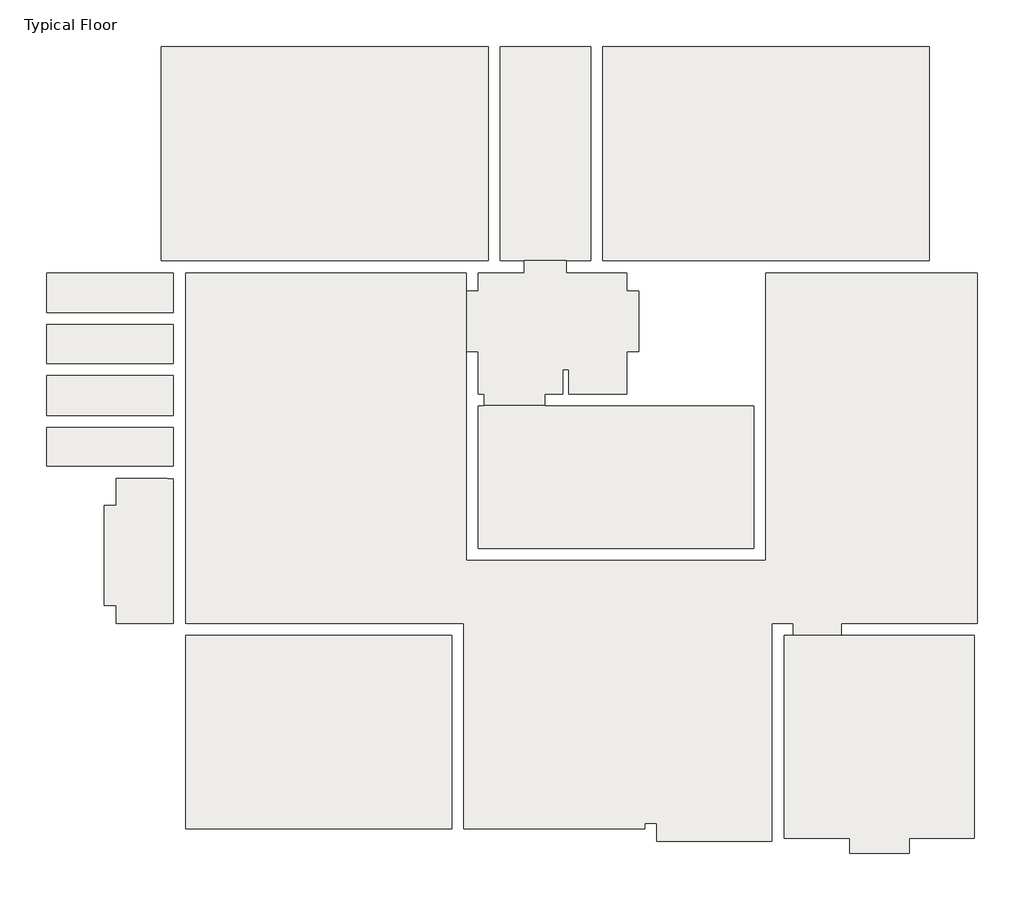
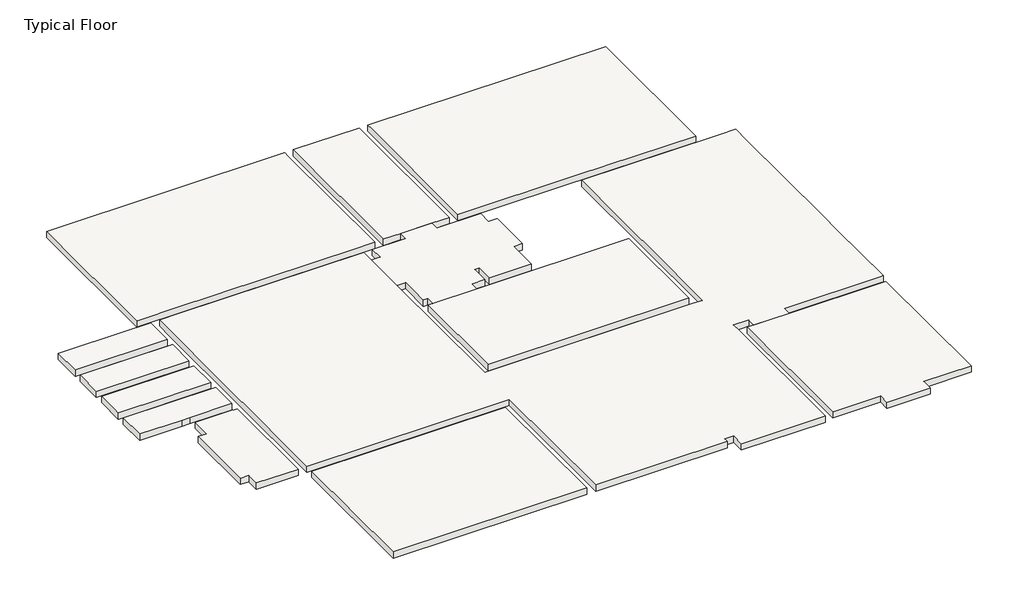
# One storey: 13 slabs.
"""IFC4 building model written with IfcOpenShell, lengths in millimetres."""

from ifc_helpers import new_model, si_unit, frame, origin, place, context, project, spatial, polyline, outline, extrude, faceted_brep, element, save

model = new_model("IFC4")

# Units and contexts
model_context = context("Model", 3, world=origin())
ifc_project = project(units=[si_unit("LENGTHUNIT", "METRE", prefix="MILLI")], contexts=[model_context])

# Site, building, storey
site = spatial("IfcSite", under=ifc_project)
building = spatial("IfcBuilding", under=site)
storey = spatial("IfcBuildingStorey", under=building, Name="Typical Floor", Elevation=3000.0)

# Slabs
placement = place(None, origin())
element("IfcSlab", 1, ObjectType="15", at=placement, inside=storey, context=model_context, shape_type="Brep", body=[
    faceted_brep([(623.0052446, -1951.586272, 2850.0), (623.0052446, 1403.8860569, 2850.0), (773.8332228, 1403.8860569, 2850.0), (1572.9542214, 1403.8860569, 2850.0), (3773.240421, 1403.8860569, 2850.0), (3773.240421, -1951.586272, 2850.0), (2697.5461186, -1951.586272, 2850.0), (2697.5461186, -2201.586272, 2850.0), (1713.8332228, -2201.586272, 2850.0), (1713.8332228, -1951.586272, 2850.0), (623.0052446, 1403.8860569, 3000.0), (623.0052446, -1951.586272, 3000.0), (1713.8332228, -1951.586272, 3000.0), (1713.8332228, -2201.586272, 3000.0), (2697.5461186, -2201.586272, 3000.0), (2697.5461186, -1951.586272, 3000.0), (3773.240421, -1951.586272, 3000.0), (3773.240421, 1403.8860569, 3000.0), (1572.9542214, 1403.8860569, 3000.0), (773.8332228, 1403.8860569, 3000.0)], [[[0, 1, 2, 3, 4, 5, 6, 7, 8, 9]], [[10, 11, 12, 13, 14, 15, 16, 17, 18, 19]], [[1, 0, 11, 10]], [[4, 3, 2, 1, 10, 19, 18, 17]], [[5, 4, 17, 16]], [[0, 9, 12, 11]], [[6, 5, 16, 15]], [[7, 6, 15, 14]], [[8, 7, 14, 13]], [[9, 8, 13, 12]]]),
])
element("IfcSlab", 2, ObjectType="15", at=placement, inside=storey, context=model_context, shape_type="SweptSolid", body=[
    extrude(outline(polyline([(-4877.1268931, 1403.8855607), (-4877.1268931, -1797.4530794), (-9277.1472957, -1797.4530794), (-9277.1472957, 1403.8855607), (-4877.1268931, 1403.8855607)])), frame((0.0, 0.0, 2850.0), z_axis=(0.0, 0.0, 1.0), x_axis=(1.0, 0.0, 0.0)), (0.0, 0.0, 1.0), 150.0),
])
element("IfcSlab", 3, ObjectType="15", at=placement, inside=storey, context=model_context, shape_type="SweptSolid", body=[
    extrude(outline(polyline([(123.9972875, 2842.5882386), (-4436.0027125, 2842.5882386), (-4436.0027125, 5202.5780208), (-4335.7799232, 5202.5780208), (-4335.7799232, 5207.5780373), (-3335.5551136, 5207.5780373), (-3335.5551136, 5202.5780373), (123.9972875, 5202.5780373), (123.9972875, 2842.5882386)])), frame((0.0, 0.0, 2850.0), z_axis=(0.0, 0.0, 1.0), x_axis=(1.0, 0.0, 0.0)), (0.0, 0.0, 1.0), 150.0),
])
element("IfcSlab", 4, ObjectType="15", at=placement, inside=storey, context=model_context, shape_type="Brep", body=[
    faceted_brep([(-11576.8844551, 4205.5532536, 2850.0), (-11576.8844551, 4845.5532536, 2850.0), (-9476.8844551, 4845.5532536, 2850.0), (-9476.8844551, 4297.7532903, 2850.0), (-9476.8844551, 4205.5532536, 2850.0), (-10423.025528, 4205.5532536, 2850.0), (-10423.025528, 4208.1905626, 2850.0), (-10623.025528, 4208.1905626, 2850.0), (-10623.025528, 4205.5532536, 2850.0), (-11576.8844551, 4845.5532536, 3000.0), (-11576.8844551, 4205.5532536, 3000.0), (-10623.025528, 4205.5532536, 3000.0), (-10623.025528, 4208.1905626, 3000.0), (-10423.025528, 4208.1905626, 3000.0), (-10423.025528, 4205.5532536, 3000.0), (-9476.8844551, 4205.5532536, 3000.0), (-9476.8844551, 4297.7532903, 3000.0), (-9476.8844551, 4845.5532536, 3000.0)], [[[0, 1, 2, 3, 4, 5, 6, 7, 8]], [[9, 10, 11, 12, 13, 14, 15, 16, 17]], [[15, 4, 3, 2, 17, 16]], [[4, 15, 14, 5]], [[10, 0, 8, 11]], [[1, 0, 10, 9]], [[2, 1, 9, 17]], [[13, 6, 5, 14]], [[7, 12, 11, 8]], [[12, 7, 6, 13]]]),
])
element("IfcSlab", 5, ObjectType="15", at=placement, inside=storey, context=model_context, shape_type="SweptSolid", body=[
    extrude(outline(polyline([(-9476.8844551, 5705.5532536), (-9476.8844551, 5045.5532536), (-11576.8844551, 5045.5532536), (-11576.8844551, 5705.5532536), (-9476.8844551, 5705.5532536)])), frame((0.0, 0.0, 2850.0), z_axis=(0.0, 0.0, 1.0), x_axis=(1.0, 0.0, 0.0)), (0.0, 0.0, 1.0), 150.0),
])
element("IfcSlab", 6, ObjectType="15", at=placement, inside=storey, context=model_context, shape_type="SweptSolid", body=[
    extrude(outline(polyline([(-9476.8844551, 6545.5532536), (-9476.8844551, 5905.5532536), (-11576.8844551, 5905.5532536), (-11576.8844551, 6545.5532536), (-9476.8844551, 6545.5532536)])), frame((0.0, 0.0, 2850.0), z_axis=(0.0, 0.0, 1.0), x_axis=(1.0, 0.0, 0.0)), (0.0, 0.0, 1.0), 150.0),
])
element("IfcSlab", 7, ObjectType="15", at=placement, inside=storey, context=model_context, shape_type="Brep", body=[
    faceted_brep([(-9476.8844551, 7405.5532536, 2850.0), (-9476.8844551, 6745.5532536, 2850.0), (-11576.8844551, 6745.5532536, 2850.0), (-11576.8844551, 7405.5532536, 2850.0), (-9476.8844551, 7405.5532536, 3000.0), (-9682.6961091, 7405.5532536, 3000.0), (-9932.6961091, 7405.5532536, 3000.0), (-11576.8844551, 7405.5532536, 3000.0), (-11576.8844551, 6745.5532536, 3000.0), (-9476.8844551, 6745.5532536, 3000.0), (-9476.8844551, 7005.5532536, 3000.0)], [[[0, 1, 2, 3]], [[4, 5, 6, 7, 8, 9, 10]], [[1, 0, 4, 10, 9]], [[2, 1, 9, 8]], [[3, 2, 8, 7]], [[0, 3, 7, 6, 5, 4]]]),
])
element("IfcSlab", 8, ObjectType="15", at=placement, inside=storey, context=model_context, shape_type="Brep", body=[
    faceted_brep([(3026.9297982, 11151.9234339, 2850.0), (3026.9297982, 7605.5532536, 2850.0), (-2375.600893, 7605.5532536, 2850.0), (-2375.600893, 11151.9234339, 2850.0), (3026.9297982, 11151.9234339, 3000.0), (-2375.600893, 11151.9234339, 3000.0), (-2375.600893, 11003.3317688, 3000.0), (-2375.600893, 7605.5532536, 3000.0), (323.9972875, 7605.5532536, 3000.0), (3026.9297982, 7605.5532536, 3000.0), (3026.9297982, 11001.5732233, 3000.0)], [[[0, 1, 2, 3]], [[4, 5, 6, 7, 8, 9, 10]], [[1, 0, 4, 10, 9]], [[2, 1, 9, 8, 7]], [[3, 2, 7, 6, 5]], [[0, 3, 5, 4]]]),
])
element("IfcSlab", 9, ObjectType="15", at=placement, inside=storey, context=model_context, shape_type="Brep", body=[
    faceted_brep([(-2575.600893, 11151.9234339, 2850.0), (-2575.600893, 7605.5532536, 2850.0), (-2975.6858924, 7605.5532536, 2850.0), (-3676.9016865, 7605.5532536, 2850.0), (-4072.3731245, 7605.5532536, 2850.0), (-4072.3731245, 11151.9234339, 2850.0), (-2575.600893, 11151.9234339, 3000.0), (-4072.3731245, 11151.9234339, 3000.0), (-4072.3731245, 11003.3317688, 3000.0), (-4072.3731245, 7605.5532536, 3000.0), (-3676.9016865, 7605.5532536, 3000.0), (-2975.6858924, 7605.5532536, 3000.0), (-2575.600893, 7605.5532536, 3000.0), (-2575.600893, 11003.3317688, 3000.0)], [[[0, 1, 2, 3, 4, 5]], [[6, 7, 8, 9, 10, 11, 12, 13]], [[1, 0, 6, 13, 12]], [[4, 3, 2, 1, 12, 11, 10, 9]], [[5, 4, 9, 8, 7]], [[0, 5, 7, 6]]]),
])
element("IfcSlab", 10, ObjectType="15", at=placement, inside=storey, context=model_context, shape_type="Brep", body=[
    faceted_brep([(-4272.3731245, 11151.9234339, 2850.0), (-4272.3731245, 7605.5532536, 2850.0), (-9682.6961091, 7605.5532536, 2850.0), (-9682.6961091, 11151.9234339, 2850.0), (-4272.3731245, 11151.9234339, 3000.0), (-9682.6961091, 11151.9234339, 3000.0), (-9682.6961091, 11001.5732233, 3000.0), (-9682.6961091, 7605.5532536, 3000.0), (-9476.8844551, 7605.5532536, 3000.0), (-8876.8844551, 7605.5532536, 3000.0), (-4636.0027125, 7605.5532536, 3000.0), (-4436.0027125, 7605.5532536, 3000.0), (-4272.3731245, 7605.5532536, 3000.0), (-4272.3731245, 11003.3317688, 3000.0)], [[[0, 1, 2, 3]], [[4, 5, 6, 7, 8, 9, 10, 11, 12, 13]], [[1, 0, 4, 13, 12]], [[2, 1, 12, 11, 10, 9, 8, 7]], [[3, 2, 7, 6, 5]], [[0, 3, 5, 4]]]),
])
element("IfcSlab", 11, ObjectType="15", at=placement, inside=storey, context=model_context, shape_type="SweptSolid", body=[
    extrude(outline(polyline([(-2975.6858924, 7605.5532536), (-2975.6858924, 7405.5532536), (-1977.004444, 7405.5532536), (-1977.004444, 7102.4758421), (-1777.004444, 7102.4758421), (-1777.004444, 6104.8971794), (-1977.004444, 6104.8971794), (-1977.004444, 5402.5780373), (-2935.9943496, 5402.5780373), (-2935.9943496, 5803.2422484), (-3035.9943496, 5803.2422484), (-3035.9943496, 5402.5780373), (-3335.5551136, 5402.5780373), (-3335.5551136, 5207.5780373), (-4335.7799232, 5207.5780373), (-4335.7799232, 5402.5780208), (-4436.0027125, 5402.5780208), (-4436.0027125, 6102.5882386), (-4636.0027125, 6102.5882386), (-4636.0027125, 7102.4759909), (-4436.0027125, 7102.4759909), (-4436.0027125, 7405.5532536), (-3676.9016865, 7405.5532536), (-3676.9016865, 7605.5532536), (-2975.6858924, 7605.5532536)])), frame((0.0, 0.0, 2850.0), z_axis=(0.0, 0.0, 1.0), x_axis=(1.0, 0.0, 0.0)), (0.0, 0.0, 1.0), 150.0),
])
element("IfcSlab", 12, ObjectType="15", at=placement, inside=storey, context=model_context, shape_type="Brep", body=[
    faceted_brep([(323.9972875, 2642.5882386, 2850.0), (323.9972875, 7405.5532536, 2850.0), (3423.240421, 7405.5532536, 2850.0), (3823.240421, 7405.5532536, 2850.0), (3823.240421, 7005.5532536, 2850.0), (3823.240421, 1603.8858088, 2850.0), (3773.240421, 1603.8858088, 2850.0), (1572.9542214, 1603.8858088, 2850.0), (1572.9542214, 1403.8858088, 2850.0), (773.8332228, 1403.8858088, 2850.0), (773.8332228, 1603.8860569, 2850.0), (423.0052446, 1603.8860569, 2850.0), (423.0052446, 1403.8860569, 2850.0), (423.0052446, -2001.586272, 2850.0), (-1481.0647566, -2001.586272, 2850.0), (-1481.0647566, -1701.586272, 2850.0), (-1681.0647566, -1701.586272, 2850.0), (-1681.0647566, -1797.4530794, 2850.0), (-4677.1268931, -1797.4530794, 2850.0), (-4677.1268931, 1603.8855607, 2850.0), (-4877.1268931, 1603.8855607, 2850.0), (-9276.8844551, 1603.8855607, 2850.0), (-9276.8844551, 7005.5532536, 2850.0), (-9276.8844551, 7405.5532536, 2850.0), (-8876.8844551, 7405.5532536, 2850.0), (-4636.0027125, 7405.5532536, 2850.0), (-4636.0027125, 7102.4759909, 2850.0), (-4636.0027125, 6102.5882386, 2850.0), (-4636.0027125, 2842.5882386, 2850.0), (-4636.0027125, 2642.5882386, 2850.0), (123.9972875, 2642.5882386, 2850.0), (323.9972875, 7405.5532536, 3000.0), (323.9972875, 2642.5882386, 3000.0), (123.9972875, 2642.5882386, 3000.0), (-4636.0027125, 2642.5882386, 3000.0), (-4636.0027125, 2842.5882386, 3000.0), (-4636.0027125, 6102.5882386, 3000.0), (-4636.0027125, 7102.4759909, 3000.0), (-4636.0027125, 7405.5532536, 3000.0), (-8876.8844551, 7405.5532536, 3000.0), (-9276.8844551, 7405.5532536, 3000.0), (-9276.8844551, 7005.5532536, 3000.0), (-9276.8844551, 4297.7532903, 3000.0), (-9276.8844551, 3997.7532903, 3000.0), (-9276.8844551, 1603.8855607, 3000.0), (-4877.1268931, 1603.8855607, 3000.0), (-4677.1268931, 1603.8855607, 3000.0), (-4677.1268931, -1797.4530794, 3000.0), (-1681.0647566, -1797.4530794, 3000.0), (-1681.0647566, -1701.586272, 3000.0), (-1481.0647566, -1701.586272, 3000.0), (-1481.0647566, -2001.586272, 3000.0), (423.0052446, -2001.586272, 3000.0), (423.0052446, 1403.8860569, 3000.0), (423.0052446, 1603.8860569, 3000.0), (773.8332228, 1603.8860569, 3000.0), (773.8332228, 1403.8858088, 3000.0), (1572.9542214, 1403.8858088, 3000.0), (1572.9542214, 1603.8858088, 3000.0), (3773.240421, 1603.8858088, 3000.0), (3823.240421, 1603.8858088, 3000.0), (3823.240421, 3398.9311809, 3000.0), (3823.240421, 3998.9311809, 3000.0), (3823.240421, 7005.5532536, 3000.0), (3823.240421, 7405.5532536, 3000.0), (3423.240421, 7405.5532536, 3000.0)], [[[0, 1, 2, 3, 4, 5, 6, 7, 8, 9, 10, 11, 12, 13, 14, 15, 16, 17, 18, 19, 20, 21, 22, 23, 24, 25, 26, 27, 28, 29, 30]], [[31, 32, 33, 34, 35, 36, 37, 38, 39, 40, 41, 42, 43, 44, 45, 46, 47, 48, 49, 50, 51, 52, 53, 54, 55, 56, 57, 58, 59, 60, 61, 62, 63, 64, 65]], [[34, 29, 28, 27, 26, 25, 38, 37, 36, 35]], [[29, 34, 33, 32, 0, 30]], [[1, 0, 32, 31]], [[1, 31, 65, 64, 3, 2]], [[3, 64, 63, 62, 61, 60, 5, 4]], [[5, 60, 59, 58, 7, 6]], [[8, 7, 58, 57]], [[9, 8, 57, 56]], [[10, 9, 56, 55]], [[11, 10, 55, 54]], [[11, 54, 53, 52, 13, 12]], [[14, 13, 52, 51]], [[15, 14, 51, 50]], [[16, 15, 50, 49]], [[17, 16, 49, 48]], [[18, 17, 48, 47]], [[19, 18, 47, 46]], [[19, 46, 45, 44, 21, 20]], [[21, 44, 43, 42, 41, 40, 23, 22]], [[23, 40, 39, 38, 25, 24]]]),
])
element("IfcSlab", 13, ObjectType="15", at=placement, inside=storey, context=model_context, shape_type="Brep", body=[
    faceted_brep([(-9476.8844551, 1603.8855607, 2850.0), (-10423.025528, 1603.8855607, 2850.0), (-10423.025528, 1900.4395709, 2850.0), (-10623.025528, 1900.4395709, 2850.0), (-10623.025528, 3558.1905626, 2850.0), (-10423.025528, 3558.1905626, 2850.0), (-10423.025528, 4005.5532536, 2850.0), (-9576.8844551, 4005.5532536, 2850.0), (-9576.8844551, 3997.7532903, 2850.0), (-9476.8844551, 3997.7532903, 2850.0), (-10423.025528, 1603.8855607, 3000.0), (-9477.1472957, 1603.8855607, 3000.0), (-9476.8844551, 1603.8855607, 3000.0), (-9476.8844551, 3997.7532903, 3000.0), (-9576.8844551, 3997.7532903, 3000.0), (-9576.8844551, 4005.5532536, 3000.0), (-10423.025528, 4005.5532536, 3000.0), (-10423.025528, 3558.1905626, 3000.0), (-10623.025528, 3558.1905626, 3000.0), (-10623.025528, 1900.4395709, 3000.0), (-10423.025528, 1900.4395709, 3000.0)], [[[0, 1, 2, 3, 4, 5, 6, 7, 8, 9]], [[10, 11, 12, 13, 14, 15, 16, 17, 18, 19, 20]], [[12, 0, 9, 13]], [[1, 0, 12, 11, 10]], [[2, 1, 10, 20]], [[3, 2, 20, 19]], [[4, 3, 19, 18]], [[5, 4, 18, 17]], [[6, 5, 17, 16]], [[6, 16, 15, 7]], [[8, 14, 13, 9]], [[14, 8, 7, 15]]]),
])

save(model, "model.ifc")

# Revit data of these elements
# Type "15"
#   Function = 0
#   Layers, outside or top first: 15 cm "Concrete" (function 1)
# Element 1 (IfcSlab, "15")
#   Mark = "S1"
#   SOFiSTiK_AMG_Comments = ""
#   built-in parameter 1001955 = 3.14159 (stored number, unit not read)
#   Height Offset From Level = 0 cm
#   built-in parameter 1001954 = 1
#   SOFiSTiK_AMG_Scheduled = yes
#   SOFiSTiK_AMG_Adjusted = yes
#   Phase Created = New Construction
#   Materials on its faces: "Concrete"
# Element 2 (IfcSlab, "15")
#   Mark = "S2"
#   SOFiSTiK_AMG_Comments = ""
#   Height Offset From Level = 0 cm
#   built-in parameter 1001954 = 1
#   SOFiSTiK_AMG_Scheduled = yes
#   SOFiSTiK_AMG_Adjusted = yes
#   Phase Created = New Construction
#   Materials on its faces: "Concrete"
# Element 3 (IfcSlab, "15")
#   Mark = "S3"
#   SOFiSTiK_AMG_Comments = ""
#   Height Offset From Level = 0 cm
#   built-in parameter 1001954 = 1
#   SOFiSTiK_AMG_Scheduled = yes
#   SOFiSTiK_AMG_Adjusted = yes
#   Phase Created = New Construction
#   Materials on its faces: "Concrete"
# Element 4 (IfcSlab, "15")
#   Mark = "S4"
#   SOFiSTiK_AMG_Comments = ""
#   Height Offset From Level = 0 cm
#   built-in parameter 1001954 = 1
#   SOFiSTiK_AMG_Scheduled = yes
#   SOFiSTiK_AMG_Adjusted = yes
#   Phase Created = New Construction
#   Materials on its faces: "Concrete"
# Element 5 (IfcSlab, "15")
#   Mark = "S5"
#   SOFiSTiK_AMG_Comments = ""
#   Height Offset From Level = 0 cm
#   built-in parameter 1001954 = 1
#   SOFiSTiK_AMG_Scheduled = yes
#   SOFiSTiK_AMG_Adjusted = yes
#   Phase Created = New Construction
#   Materials on its faces: "Concrete"
# Element 6 (IfcSlab, "15")
#   Mark = "S6"
#   SOFiSTiK_AMG_Comments = ""
#   Height Offset From Level = 0 cm
#   built-in parameter 1001954 = 1
#   SOFiSTiK_AMG_Scheduled = yes
#   SOFiSTiK_AMG_Adjusted = yes
#   Phase Created = New Construction
#   Materials on its faces: "Concrete"
# Element 7 (IfcSlab, "15")
#   Mark = "S7"
#   SOFiSTiK_AMG_Comments = ""
#   Height Offset From Level = 0 cm
#   built-in parameter 1001954 = 1
#   SOFiSTiK_AMG_Scheduled = yes
#   SOFiSTiK_AMG_Adjusted = yes
#   Phase Created = New Construction
#   Materials on its faces: "Concrete"
# Element 8 (IfcSlab, "15")
#   Mark = "S8"
#   SOFiSTiK_AMG_Comments = ""
#   Height Offset From Level = 0 cm
#   built-in parameter 1001954 = 1
#   SOFiSTiK_AMG_Scheduled = yes
#   SOFiSTiK_AMG_Adjusted = yes
#   Phase Created = New Construction
#   Materials on its faces: "Concrete"
# Element 9 (IfcSlab, "15")
#   Mark = "S9"
#   SOFiSTiK_AMG_Comments = ""
#   Height Offset From Level = 0 cm
#   built-in parameter 1001954 = 1
#   SOFiSTiK_AMG_Scheduled = yes
#   SOFiSTiK_AMG_Adjusted = yes
#   Phase Created = New Construction
#   Materials on its faces: "Concrete"
# Element 10 (IfcSlab, "15")
#   Mark = "S10"
#   SOFiSTiK_AMG_Comments = ""
#   Height Offset From Level = 0 cm
#   built-in parameter 1001954 = 1
#   SOFiSTiK_AMG_Scheduled = yes
#   SOFiSTiK_AMG_Adjusted = yes
#   Phase Created = New Construction
#   Materials on its faces: "Concrete"
# Element 11 (IfcSlab, "15")
#   Mark = "S11"
#   SOFiSTiK_AMG_Comments = ""
#   Height Offset From Level = 0 cm
#   built-in parameter 1001954 = 1
#   SOFiSTiK_AMG_Scheduled = yes
#   SOFiSTiK_AMG_Adjusted = yes
#   Phase Created = New Construction
#   Materials on its faces: "Concrete"
# Element 12 (IfcSlab, "15")
#   Mark = "S12"
#   SOFiSTiK_AMG_Comments = ""
#   Height Offset From Level = 0 cm
#   built-in parameter 1001954 = 1
#   SOFiSTiK_AMG_Scheduled = yes
#   SOFiSTiK_AMG_Adjusted = no
#   Phase Created = New Construction
#   Materials on its faces: "Concrete"
# Element 13 (IfcSlab, "15")
#   Mark = "S13"
#   SOFiSTiK_AMG_Comments = ""
#   Height Offset From Level = 0 cm
#   built-in parameter 1001954 = 1
#   SOFiSTiK_AMG_Scheduled = yes
#   SOFiSTiK_AMG_Adjusted = yes
#   Phase Created = New Construction
#   Materials on its faces: "Concrete"
# Materials
#   "Concrete": class "Concrete", colour RGB 192 192 192, transparency 0, Keynote = "01000", Description = "Cast-in-place concrete", Cost = 0
